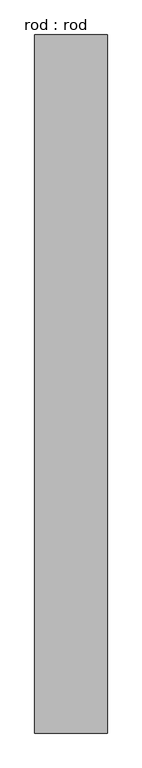
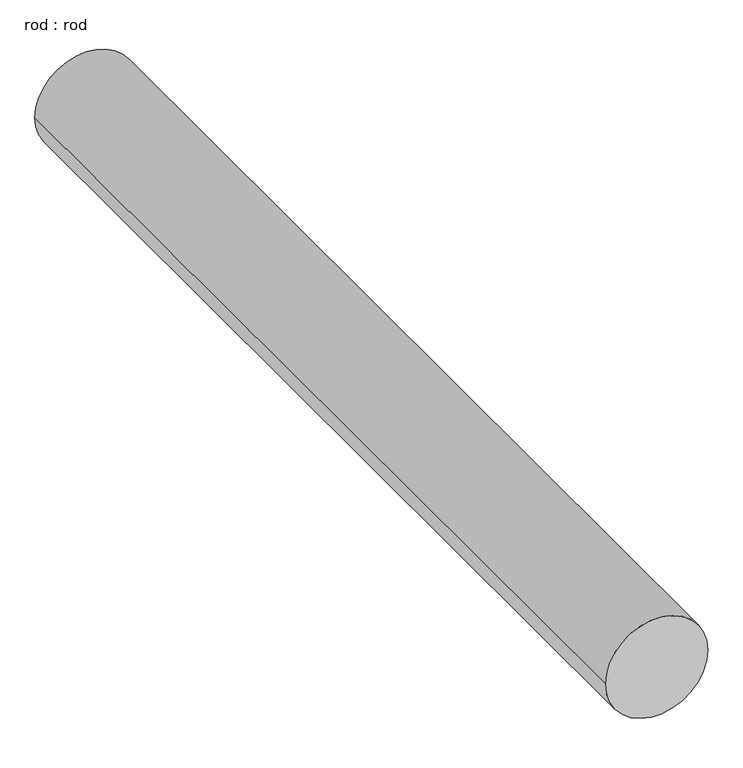
"""IFC4 building model written with IfcOpenShell, lengths in millimetres: proxy geometry, rod : rod."""

from ifc_helpers import new_model, si_unit, point, frame, frame_2d, origin, place, context, project, spatial, circle_curve, trimmed, segment, composite_curve, outline, extrude, source, transform, mapped, element, save


def rod_rod_db1fddbe(model_context):
    return source(origin(), model_context, "Body", "SweptSolid", [
        extrude(outline(composite_curve([segment(trimmed(circle_curve(frame_2d((0.0108462, 0.0)), 200.0), [point((0.0108462, 200.0))], [point((0.0108462, -200.0))], False, "CARTESIAN"), True, "CONTINUOUS"), segment(trimmed(circle_curve(frame_2d((0.0108462, 0.0)), 200.0), [point((0.0108462, -200.0))], [point((0.0108462, 200.0))], False, "CARTESIAN"), True, "CONTINUOUS")], self_intersect=False)), frame((0.0, 2169.5135338, 0.0), z_axis=(0.0, 1.0, 0.0), x_axis=(0.0, 0.0, 1.0)), (0.0, 0.0, 1.0), 3846.4301632),
    ])


if __name__ == "__main__":
    model = new_model("IFC4")
    model_context = context("Model", 3, world=origin())
    ifc_project = project(units=[si_unit("LENGTHUNIT", "METRE", prefix="MILLI")], contexts=[model_context])
    site = spatial("IfcSite", under=ifc_project)
    building = spatial("IfcBuilding", under=site)
    placement = place(None, origin())
    rod_rod_shape = rod_rod_db1fddbe(model_context)
    element("IfcBuildingElementProxy", 1, Name="rod : rod", ObjectType="rod : rod", at=placement, inside=building, context=model_context, shape_type="MappedRepresentation", body=[
        mapped(rod_rod_shape, transform((0.0, 0.0, 0.0), x_axis=(1.0, 0.0, 0.0), y_axis=(0.0, 1.0, 0.0), z_axis=(0.0, 0.0, 1.0))),
    ])
    save(model, "model.ifc")

# Revit data of these elements
# Type "rod : rod"
#   Default Elevation = 0
